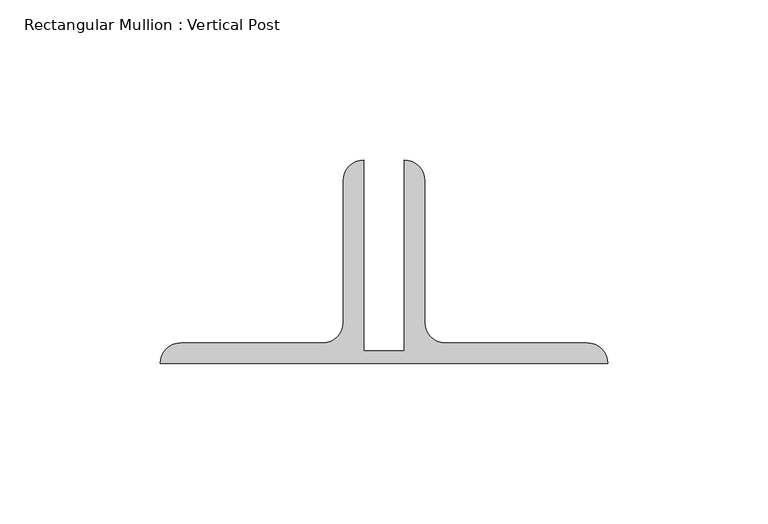
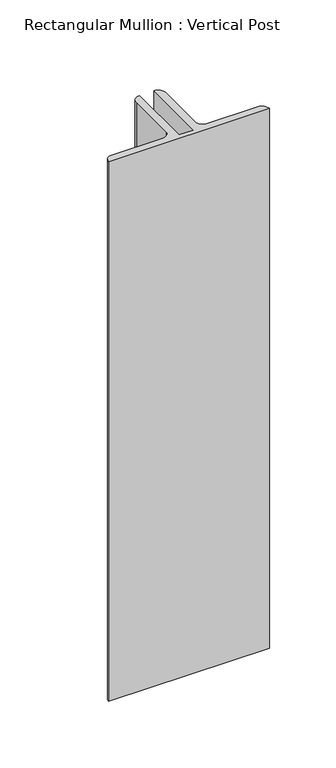
"""IFC4 building model written with IfcOpenShell, lengths in millimetres: member geometry, Rectangular Mullion : Vertical Post."""

from ifc_helpers import new_model, si_unit, point, frame, frame_2d, origin, place, context, project, spatial, polyline, circle_curve, trimmed, segment, composite_curve, outline, extrude, source, transform, mapped, element, save


def rectangular_mullion_vertical_post_21d5de07(model_context):
    return source(origin(), model_context, "Body", "SweptSolid", [
        extrude(outline(composite_curve([segment(polyline([(-6.35, 22.9145205), (6.35, 22.9145205), (6.35, 82.55)]), True, "CONTINUOUS"), segment(trimmed(circle_curve(frame_2d((6.35, 76.2)), 6.35), [point((6.35, 82.55))], [point((12.7, 76.2))], False, "CARTESIAN"), True, "CONTINUOUS"), segment(polyline([(12.7, 76.2), (12.7, 31.75)]), True, "CONTINUOUS"), segment(trimmed(circle_curve(frame_2d((19.05, 31.75)), 6.35), [point((12.7, 31.75))], [point((19.05, 25.4))], True, "CARTESIAN"), True, "CONTINUOUS"), segment(polyline([(19.05, 25.4), (63.5, 25.4)]), True, "CONTINUOUS"), segment(trimmed(circle_curve(frame_2d((63.5, 19.05)), 6.35), [point((63.5, 25.4))], [point((69.85, 19.05))], False, "CARTESIAN"), True, "CONTINUOUS"), segment(polyline([(69.85, 19.05), (-69.85, 19.05)]), True, "CONTINUOUS"), segment(trimmed(circle_curve(frame_2d((-63.5, 19.05)), 6.35), [point((-69.85, 19.05))], [point((-63.5, 25.4))], False, "CARTESIAN"), True, "CONTINUOUS"), segment(polyline([(-63.5, 25.4), (-19.05, 25.4)]), True, "CONTINUOUS"), segment(trimmed(circle_curve(frame_2d((-19.05, 31.75)), 6.35), [point((-19.05, 25.4))], [point((-12.7, 31.75))], True, "CARTESIAN"), True, "CONTINUOUS"), segment(polyline([(-12.7, 31.75), (-12.7, 76.2)]), True, "CONTINUOUS"), segment(trimmed(circle_curve(frame_2d((-6.35, 76.2)), 6.35), [point((-12.7, 76.2))], [point((-6.35, 82.55))], False, "CARTESIAN"), True, "CONTINUOUS"), segment(polyline([(-6.35, 82.55), (-6.35, 22.9145205)]), True, "CONTINUOUS")], self_intersect=False)), frame((0.0, 0.0, -495.3992188), z_axis=(0.0, 0.0, 1.0), x_axis=(1.0, 0.0, 0.0)), (0.0, 0.0, 1.0), 495.3992188),
    ])


if __name__ == "__main__":
    model = new_model("IFC4")
    model_context = context("Model", 3, world=origin())
    ifc_project = project(units=[si_unit("LENGTHUNIT", "METRE", prefix="MILLI")], contexts=[model_context])
    site = spatial("IfcSite", under=ifc_project)
    building = spatial("IfcBuilding", under=site)
    placement = place(None, origin())
    rectangular_mullion_vertical_post_shape = rectangular_mullion_vertical_post_21d5de07(model_context)
    element("IfcMember", 1, ObjectType="Rectangular Mullion : Vertical Post", at=placement, inside=building, context=model_context, shape_type="MappedRepresentation", body=[
        mapped(rectangular_mullion_vertical_post_shape, transform((0.0, 0.0, 0.0), x_axis=(1.0, 0.0, 0.0), y_axis=(0.0, 1.0, 0.0), z_axis=(0.0, 0.0, 1.0))),
    ])
    save(model, "model.ifc")

# Revit data of these elements
# Type "Rectangular Mullion : Vertical Post"
#   built-in parameter 1007351 = -0.0625 (stored number, unit not read)
#   built-in parameter 1007322 = 0.0126789 (stored number, unit not read)
#   built-in parameter 1007321 = 0.229167 (stored number, unit not read)
#   built-in parameter 1007320 = 0.229167 (stored number, unit not read)
# Element 1 (IfcMember, "Rectangular Mullion : Vertical Post")
#   Materials on its faces: "GATE POST: (2) BACK/BACK GALVANIZED ANGLES"
# Materials
#   "GATE POST: (2) BACK/BACK GALVANIZED ANGLES": class "Unassigned", colour RGB 211 211 211, transparency 0, Cost = 0
